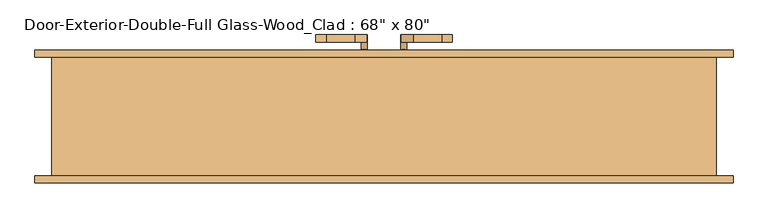
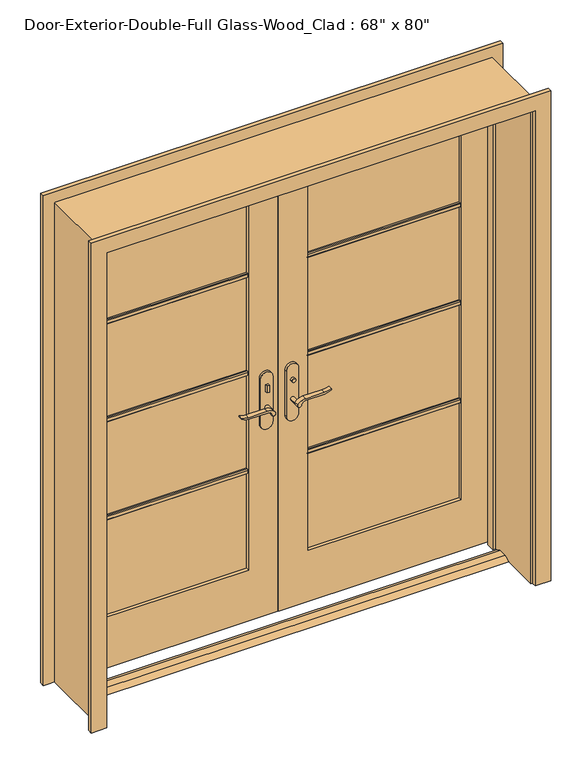
"""IFC4 building model written with IfcOpenShell, lengths in millimetres: door geometry."""

from ifc_helpers import new_model, si_unit, point, frame, frame_2d, origin, place, context, project, spatial, polyline, circle_curve, trimmed, segment, composite_curve, outline, extrude, faceted_brep, source, transform, mapped, element, save


def door_97aac55e(model_context):
    return source(origin(), model_context, "Body", "SolidModel", [
        extrude(outline(polyline([(19.05, 12.7), (53.975, 12.7), (79.375, 0.0), (-6.35, 0.0), (19.05, 12.7)])), frame((-863.6, 0.0, 0.0), z_axis=(1.0, 0.0, 0.0), x_axis=(0.0, 1.0, 0.0)), (0.0, 0.0, 1.0), 1727.2),
        extrude(outline(polyline([(-47.4019111, 100.65), (-57.4019111, 100.65), (-57.4019111, 110.65), (-47.4019111, 110.65), (-47.4019111, 100.65)])), frame((0.0, 0.0, 981.9), z_axis=(0.0, 0.0, 1.0), x_axis=(1.0, 0.0, 0.0)), (0.0, 0.0, 1.0), 30.0),
        extrude(outline(composite_curve([segment(trimmed(circle_curve(frame_2d((996.9, -52.4019111)), 8.0), [point((996.9, -60.4019111))], [point((996.9, -44.4019111))], False, "CARTESIAN"), True, "CONTINUOUS"), segment(trimmed(circle_curve(frame_2d((996.9, -52.4019111)), 8.0), [point((996.9, -44.4019111))], [point((996.9, -60.4019111))], False, "CARTESIAN"), True, "CONTINUOUS")], self_intersect=False)), frame((0.0, 165.575, 0.0), z_axis=(0.0, 1.0, 0.0), x_axis=(0.0, 0.0, 1.0)), (0.0, 0.0, 1.0), 10.0),
        extrude(outline(composite_curve([segment(trimmed(circle_curve(frame_2d((897.1555521, -76.0694241)), 37.2832219), [point((919.0523287, -45.8937749))], [point((934.4, -77.7693445))], False, "CARTESIAN"), True, "CONTINUOUS"), segment(polyline([(934.4, -77.7693445), (934.4, -154.045502)]), True, "CONTINUOUS"), segment(trimmed(circle_curve(frame_2d((1017.6850638, -153.9791202)), 83.2850902), [point((934.4, -154.045502))], [point((939.4, -182.4019111))], True, "CARTESIAN"), True, "CONTINUOUS"), segment(polyline([(939.4, -182.4019111), (936.6135558, -182.4019111)]), True, "CONTINUOUS"), segment(trimmed(circle_curve(frame_2d((986.6709207, -150.4622499)), 59.3791355), [point((936.6135558, -182.4019111))], [point((927.4, -154.045502))], False, "CARTESIAN"), True, "CONTINUOUS"), segment(polyline([(927.4, -154.045502), (927.4, -77.7881013)]), True, "CONTINUOUS"), segment(trimmed(circle_curve(frame_2d((909.2738613, -77.7881013)), 18.1261387), [point((927.4, -77.7881013))], [point((914.4, -60.4019111))], True, "CARTESIAN"), True, "CONTINUOUS"), segment(trimmed(circle_curve(frame_2d((914.4, -52.4019111)), 8.0), [point((914.4, -60.4019111))], [point((919.0523287, -45.8937749))], False, "CARTESIAN"), True, "CONTINUOUS")], self_intersect=False)), frame((0.0, 60.65, 0.0), z_axis=(0.0, 1.0, 0.0), x_axis=(0.0, 0.0, 1.0)), (0.0, 0.0, 1.0), 20.0),
        extrude(outline(composite_curve([segment(trimmed(circle_curve(frame_2d((914.4, -52.4019111)), 8.0), [point((914.3999903, -60.4019111))], [point((919.0523287, -45.8937749))], False, "CARTESIAN"), True, "CONTINUOUS"), segment(trimmed(circle_curve(frame_2d((897.1555521, -76.0694241)), 37.2832219), [point((919.0523287, -45.8937749))], [point((934.4, -77.7693445))], False, "CARTESIAN"), True, "CONTINUOUS"), segment(polyline([(934.4, -77.7693445), (934.4, -154.045502)]), True, "CONTINUOUS"), segment(trimmed(circle_curve(frame_2d((1017.6850638, -153.9791202)), 83.2850902), [point((934.4, -154.045502))], [point((939.4, -182.4019111))], True, "CARTESIAN"), True, "CONTINUOUS"), segment(polyline([(939.4, -182.4019111), (936.6135558, -182.4019111)]), True, "CONTINUOUS"), segment(trimmed(circle_curve(frame_2d((986.6709207, -150.4622499)), 59.3791355), [point((936.6135558, -182.4019111))], [point((927.4, -154.045502))], False, "CARTESIAN"), True, "CONTINUOUS"), segment(polyline([(927.4, -154.045502), (927.4, -77.788099)]), True, "CONTINUOUS"), segment(trimmed(circle_curve(frame_2d((909.2738682, -77.788099)), 18.1261318), [point((927.4, -77.788099))], [point((914.3999903, -60.4019111))], True, "CARTESIAN"), True, "CONTINUOUS")], self_intersect=False)), frame((0.0, 195.575, 0.0), z_axis=(0.0, 1.0, 0.0), x_axis=(0.0, 0.0, 1.0)), (0.0, 0.0, 1.0), 20.0),
        extrude(outline(composite_curve([segment(trimmed(circle_curve(frame_2d((914.4, -52.4019111)), 8.0), [point((914.4, -60.4019111))], [point((914.4, -44.4019111))], False, "CARTESIAN"), True, "CONTINUOUS"), segment(trimmed(circle_curve(frame_2d((914.4, -52.4019111)), 8.0), [point((914.4, -44.4019111))], [point((914.4, -60.4019111))], False, "CARTESIAN"), True, "CONTINUOUS")], self_intersect=False)), frame((0.0, 80.65, 0.0), z_axis=(0.0, 1.0, 0.0), x_axis=(0.0, 0.0, 1.0)), (0.0, 0.0, 1.0), 30.0),
        extrude(outline(composite_curve([segment(trimmed(circle_curve(frame_2d((914.4, -52.4019111)), 8.0), [point((914.4, -60.4019111))], [point((914.4, -44.4019111))], False, "CARTESIAN"), True, "CONTINUOUS"), segment(trimmed(circle_curve(frame_2d((914.4, -52.4019111)), 8.0), [point((914.4, -44.4019111))], [point((914.4, -60.4019111))], False, "CARTESIAN"), True, "CONTINUOUS")], self_intersect=False)), frame((0.0, 165.575, 0.0), z_axis=(0.0, 1.0, 0.0), x_axis=(0.0, 0.0, 1.0)), (0.0, 0.0, 1.0), 30.0),
        extrude(outline(composite_curve([segment(polyline([(844.4, -27.4019111), (1039.4, -27.4019111)]), True, "CONTINUOUS"), segment(trimmed(circle_curve(frame_2d((1039.4, -52.4019111)), 25.0), [point((1039.4, -27.4019111))], [point((1039.4, -77.4019111))], False, "CARTESIAN"), True, "CONTINUOUS"), segment(polyline([(1039.4, -77.4019111), (844.4, -77.4019111)]), True, "CONTINUOUS"), segment(trimmed(circle_curve(frame_2d((844.4, -52.4019111)), 25.0), [point((844.4, -77.4019111))], [point((844.4, -27.4019111))], False, "CARTESIAN"), True, "CONTINUOUS")], self_intersect=False)), frame((0.0, 110.65, 0.0), z_axis=(0.0, 1.0, 0.0), x_axis=(0.0, 0.0, 1.0)), (0.0, 0.0, 1.0), 10.0),
        extrude(outline(composite_curve([segment(polyline([(844.4, -27.4019111), (1039.4, -27.4019111)]), True, "CONTINUOUS"), segment(trimmed(circle_curve(frame_2d((1039.4, -52.4019111)), 25.0), [point((1039.4, -27.4019111))], [point((1039.4, -77.4019111))], False, "CARTESIAN"), True, "CONTINUOUS"), segment(polyline([(1039.4, -77.4019111), (844.4, -77.4019111)]), True, "CONTINUOUS"), segment(trimmed(circle_curve(frame_2d((844.4, -52.4019111)), 25.0), [point((844.4, -77.4019111))], [point((844.4, -27.4019111))], False, "CARTESIAN"), True, "CONTINUOUS")], self_intersect=False)), frame((0.0, 155.575, 0.0), z_axis=(0.0, 1.0, 0.0), x_axis=(0.0, 0.0, 1.0)), (0.0, 0.0, 1.0), 10.0),
        extrude(outline(polyline([(47.3875, 175.575), (57.3875, 175.575), (57.3875, 165.575), (47.3875, 165.575), (47.3875, 175.575)])), frame((0.0, 0.0, 981.9), z_axis=(0.0, 0.0, 1.0), x_axis=(1.0, 0.0, 0.0)), (0.0, 0.0, 1.0), 30.0),
        extrude(outline(composite_curve([segment(trimmed(circle_curve(frame_2d((996.9, 52.3875)), 8.0), [point((996.9, 60.3875))], [point((996.9, 44.3875))], False, "CARTESIAN"), True, "CONTINUOUS"), segment(trimmed(circle_curve(frame_2d((996.9, 52.3875)), 8.0), [point((996.9, 44.3875))], [point((996.9, 60.3875))], False, "CARTESIAN"), True, "CONTINUOUS")], self_intersect=False)), frame((0.0, 100.65, 0.0), z_axis=(0.0, 1.0, 0.0), x_axis=(0.0, 0.0, 1.0)), (0.0, 0.0, 1.0), 10.0),
        extrude(outline(composite_curve([segment(trimmed(circle_curve(frame_2d((914.4, 52.3875)), 8.0), [point((919.0523287, 45.8793637))], [point((914.4, 60.3875))], False, "CARTESIAN"), True, "CONTINUOUS"), segment(trimmed(circle_curve(frame_2d((909.2738613, 77.7736901)), 18.1261387), [point((914.4, 60.3875))], [point((927.4, 77.7736901))], True, "CARTESIAN"), True, "CONTINUOUS"), segment(polyline([(927.4, 77.7736901), (927.4, 154.0310909)]), True, "CONTINUOUS"), segment(trimmed(circle_curve(frame_2d((986.6709207, 150.4478388)), 59.3791355), [point((927.4, 154.0310909))], [point((936.6135558, 182.3875))], False, "CARTESIAN"), True, "CONTINUOUS"), segment(polyline([(936.6135558, 182.3875), (939.4, 182.3875)]), True, "CONTINUOUS"), segment(trimmed(circle_curve(frame_2d((1017.6850638, 153.9647091)), 83.2850902), [point((939.4, 182.3875))], [point((934.4, 154.0310909))], True, "CARTESIAN"), True, "CONTINUOUS"), segment(polyline([(934.4, 154.0310909), (934.4, 77.7549333)]), True, "CONTINUOUS"), segment(trimmed(circle_curve(frame_2d((897.1555521, 76.0550129)), 37.2832219), [point((934.4, 77.7549333))], [point((919.0523287, 45.8793637))], False, "CARTESIAN"), True, "CONTINUOUS")], self_intersect=False)), frame((0.0, 195.575, 0.0), z_axis=(0.0, 1.0, 0.0), x_axis=(0.0, 0.0, 1.0)), (0.0, 0.0, 1.0), 20.0),
        extrude(outline(composite_curve([segment(trimmed(circle_curve(frame_2d((909.2738682, 77.7736878)), 18.1261318), [point((914.3999903, 60.3875))], [point((927.4, 77.7736878))], True, "CARTESIAN"), True, "CONTINUOUS"), segment(polyline([(927.4, 77.7736878), (927.4, 154.0310909)]), True, "CONTINUOUS"), segment(trimmed(circle_curve(frame_2d((986.6709207, 150.4478388)), 59.3791355), [point((927.4, 154.0310909))], [point((936.6135558, 182.3875))], False, "CARTESIAN"), True, "CONTINUOUS"), segment(polyline([(936.6135558, 182.3875), (939.4, 182.3875)]), True, "CONTINUOUS"), segment(trimmed(circle_curve(frame_2d((1017.6850638, 153.9647091)), 83.2850902), [point((939.4, 182.3875))], [point((934.4, 154.0310909))], True, "CARTESIAN"), True, "CONTINUOUS"), segment(polyline([(934.4, 154.0310909), (934.4, 77.7549333)]), True, "CONTINUOUS"), segment(trimmed(circle_curve(frame_2d((897.1555521, 76.0550129)), 37.2832219), [point((934.4, 77.7549333))], [point((919.0523287, 45.8793637))], False, "CARTESIAN"), True, "CONTINUOUS"), segment(trimmed(circle_curve(frame_2d((914.4, 52.3875)), 8.0), [point((919.0523287, 45.8793637))], [point((914.3999903, 60.3875))], False, "CARTESIAN"), True, "CONTINUOUS")], self_intersect=False)), frame((0.0, 60.65, 0.0), z_axis=(0.0, 1.0, 0.0), x_axis=(0.0, 0.0, 1.0)), (0.0, 0.0, 1.0), 20.0),
        extrude(outline(composite_curve([segment(trimmed(circle_curve(frame_2d((914.4, 52.3875)), 8.0), [point((914.4, 60.3875))], [point((914.4, 44.3875))], False, "CARTESIAN"), True, "CONTINUOUS"), segment(trimmed(circle_curve(frame_2d((914.4, 52.3875)), 8.0), [point((914.4, 44.3875))], [point((914.4, 60.3875))], False, "CARTESIAN"), True, "CONTINUOUS")], self_intersect=False)), frame((0.0, 165.575, 0.0), z_axis=(0.0, 1.0, 0.0), x_axis=(0.0, 0.0, 1.0)), (0.0, 0.0, 1.0), 30.0),
        extrude(outline(composite_curve([segment(trimmed(circle_curve(frame_2d((914.4, 52.3875)), 8.0), [point((914.4, 60.3875))], [point((914.4, 44.3875))], False, "CARTESIAN"), True, "CONTINUOUS"), segment(trimmed(circle_curve(frame_2d((914.4, 52.3875)), 8.0), [point((914.4, 44.3875))], [point((914.4, 60.3875))], False, "CARTESIAN"), True, "CONTINUOUS")], self_intersect=False)), frame((0.0, 80.65, 0.0), z_axis=(0.0, 1.0, 0.0), x_axis=(0.0, 0.0, 1.0)), (0.0, 0.0, 1.0), 30.0),
        extrude(outline(composite_curve([segment(trimmed(circle_curve(frame_2d((844.4, 52.3875)), 25.0), [point((844.4, 27.3875))], [point((844.4, 77.3875))], False, "CARTESIAN"), True, "CONTINUOUS"), segment(polyline([(844.4, 77.3875), (1039.4, 77.3875)]), True, "CONTINUOUS"), segment(trimmed(circle_curve(frame_2d((1039.4, 52.3875)), 25.0), [point((1039.4, 77.3875))], [point((1039.4, 27.3875))], False, "CARTESIAN"), True, "CONTINUOUS"), segment(polyline([(1039.4, 27.3875), (844.4, 27.3875)]), True, "CONTINUOUS")], self_intersect=False)), frame((0.0, 155.575, 0.0), z_axis=(0.0, 1.0, 0.0), x_axis=(0.0, 0.0, 1.0)), (0.0, 0.0, 1.0), 10.0),
        extrude(outline(composite_curve([segment(trimmed(circle_curve(frame_2d((844.4, 52.3875)), 25.0), [point((844.4, 27.3875))], [point((844.4, 77.3875))], False, "CARTESIAN"), True, "CONTINUOUS"), segment(polyline([(844.4, 77.3875), (1039.4, 77.3875)]), True, "CONTINUOUS"), segment(trimmed(circle_curve(frame_2d((1039.4, 52.3875)), 25.0), [point((1039.4, 77.3875))], [point((1039.4, 27.3875))], False, "CARTESIAN"), True, "CONTINUOUS"), segment(polyline([(1039.4, 27.3875), (844.4, 27.3875)]), True, "CONTINUOUS")], self_intersect=False)), frame((0.0, 110.65, 0.0), z_axis=(0.0, 1.0, 0.0), x_axis=(0.0, 0.0, 1.0)), (0.0, 0.0, 1.0), 10.0),
        extrude(outline(polyline([(134.62, 1502.171875), (134.62, 1483.121875), (128.27, 1483.121875), (125.095, 1486.296875), (125.095, 1498.996875), (128.27, 1502.171875), (134.62, 1502.171875)])), frame((120.65, 0.0, 0.0), z_axis=(1.0, 0.0, 0.0), x_axis=(0.0, 1.0, 0.0)), (0.0, 0.0, 1.0), 622.3),
        extrude(outline(polyline([(134.62, 1081.88125), (134.62, 1062.83125), (128.27, 1062.83125), (125.095, 1066.00625), (125.095, 1078.70625), (128.27, 1081.88125), (134.62, 1081.88125)])), frame((120.65, 0.0, 0.0), z_axis=(1.0, 0.0, 0.0), x_axis=(0.0, 1.0, 0.0)), (0.0, 0.0, 1.0), 622.3),
        extrude(outline(polyline([(134.62, 661.590625), (134.62, 642.540625), (128.27, 642.540625), (125.095, 645.715625), (125.095, 658.415625), (128.27, 661.590625), (134.62, 661.590625)])), frame((120.65, 0.0, 0.0), z_axis=(1.0, 0.0, 0.0), x_axis=(0.0, 1.0, 0.0)), (0.0, 0.0, 1.0), 622.3),
        extrude(outline(polyline([(141.605, 1502.171875), (147.955, 1502.171875), (151.13, 1498.996875), (151.13, 1486.296875), (147.955, 1483.121875), (141.605, 1483.121875), (141.605, 1502.171875)])), frame((-742.95, 0.0, 0.0), z_axis=(1.0, 0.0, 0.0), x_axis=(0.0, 1.0, 0.0)), (0.0, 0.0, 1.0), 622.3),
        extrude(outline(polyline([(141.605, 1081.88125), (147.955, 1081.88125), (151.13, 1078.70625), (151.13, 1066.00625), (147.955, 1062.83125), (141.605, 1062.83125), (141.605, 1081.88125)])), frame((-742.95, 0.0, 0.0), z_axis=(1.0, 0.0, 0.0), x_axis=(0.0, 1.0, 0.0)), (0.0, 0.0, 1.0), 622.3),
        extrude(outline(polyline([(141.605, 661.590625), (147.955, 661.590625), (151.13, 658.415625), (151.13, 645.715625), (147.955, 642.540625), (141.605, 642.540625), (141.605, 661.590625)])), frame((-742.95, 0.0, 0.0), z_axis=(1.0, 0.0, 0.0), x_axis=(0.0, 1.0, 0.0)), (0.0, 0.0, 1.0), 622.3),
        extrude(outline(polyline([(141.605, 1502.171875), (147.955, 1502.171875), (151.13, 1498.996875), (151.13, 1486.296875), (147.955, 1483.121875), (141.605, 1483.121875), (141.605, 1502.171875)])), frame((120.65, 0.0, 0.0), z_axis=(1.0, 0.0, 0.0), x_axis=(0.0, 1.0, 0.0)), (0.0, 0.0, 1.0), 622.3),
        extrude(outline(polyline([(141.605, 1081.88125), (147.955, 1081.88125), (151.13, 1078.70625), (151.13, 1066.00625), (147.955, 1062.83125), (141.605, 1062.83125), (141.605, 1081.88125)])), frame((120.65, 0.0, 0.0), z_axis=(1.0, 0.0, 0.0), x_axis=(0.0, 1.0, 0.0)), (0.0, 0.0, 1.0), 622.3),
        extrude(outline(polyline([(141.605, 661.590625), (147.955, 661.590625), (151.13, 658.415625), (151.13, 645.715625), (147.955, 642.540625), (141.605, 642.540625), (141.605, 661.590625)])), frame((120.65, 0.0, 0.0), z_axis=(1.0, 0.0, 0.0), x_axis=(0.0, 1.0, 0.0)), (0.0, 0.0, 1.0), 622.3),
        extrude(outline(polyline([(134.62, 1502.171875), (134.62, 1483.121875), (128.27, 1483.121875), (125.095, 1486.296875), (125.095, 1498.996875), (128.27, 1502.171875), (134.62, 1502.171875)])), frame((-742.95, 0.0, 0.0), z_axis=(1.0, 0.0, 0.0), x_axis=(0.0, 1.0, 0.0)), (0.0, 0.0, 1.0), 622.3),
        extrude(outline(polyline([(134.62, 1081.88125), (134.62, 1062.83125), (128.27, 1062.83125), (125.095, 1066.00625), (125.095, 1078.70625), (128.27, 1081.88125), (134.62, 1081.88125)])), frame((-742.95, 0.0, 0.0), z_axis=(1.0, 0.0, 0.0), x_axis=(0.0, 1.0, 0.0)), (0.0, 0.0, 1.0), 622.3),
        extrude(outline(polyline([(134.62, 661.590625), (134.62, 642.540625), (128.27, 642.540625), (125.095, 645.715625), (125.095, 658.415625), (128.27, 661.590625), (134.62, 661.590625)])), frame((-742.95, 0.0, 0.0), z_axis=(1.0, 0.0, 0.0), x_axis=(0.0, 1.0, 0.0)), (0.0, 0.0, 1.0), 622.3),
        extrude(outline(polyline([(0.0, 869.95), (0.0, 933.45), (2101.85, 933.45), (2101.85, -933.45), (0.0, -933.45), (0.0, -869.95), (2038.35, -869.95), (2038.35, 869.95), (0.0, 869.95)])), frame((0.0, 155.575, 0.0), z_axis=(0.0, 1.0, 0.0), x_axis=(0.0, 0.0, 1.0)), (0.0, 0.0, 1.0), 19.05),
        extrude(outline(polyline([(0.0, 869.95), (0.0, 933.45), (2101.85, 933.45), (2101.85, -933.45), (0.0, -933.45), (0.0, -869.95), (2038.35, -869.95), (2038.35, 869.95), (0.0, 869.95)])), frame((0.0, -180.975, 0.0), z_axis=(0.0, 1.0, 0.0), x_axis=(0.0, 0.0, 1.0)), (0.0, 0.0, 1.0), 19.05),
        extrude(outline(polyline([(12.7, 863.6), (2032.0, 863.6), (2032.0, 1.5875), (12.7, 1.5875), (12.7, 863.6)]), holes=[polyline([(1912.9375, 120.65), (1912.9375, 742.95), (231.775, 742.95), (231.775, 120.65), (1912.9375, 120.65)])]), frame((0.0, 120.65, 0.0), z_axis=(0.0, 1.0, 0.0), x_axis=(0.0, 0.0, 1.0)), (0.0, 0.0, 1.0), 34.925),
        extrude(outline(polyline([(2032.0, -863.6), (12.7, -863.6), (12.7, -1.6019111), (2032.0, -1.6019111), (2032.0, -863.6)]), holes=[polyline([(231.775, -742.95), (1912.9375, -742.95), (1912.9375, -120.65), (231.775, -120.65), (231.775, -742.95)])]), frame((0.0, 120.65, 0.0), z_axis=(0.0, 1.0, 0.0), x_axis=(0.0, 0.0, 1.0)), (0.0, 0.0, 1.0), 34.925),
        faceted_brep([(889.0, 155.575, 0.0), (889.0, -161.925, 0.0), (863.6, -161.925, 0.0), (863.6, 85.725, 0.0), (850.9, 85.725, 0.0), (850.9, 120.65, 0.0), (863.6, 120.65, 0.0), (863.6, 155.575, 0.0), (889.0, 155.575, 2057.4), (889.0, -161.925, 2057.4), (-889.0, -161.925, 2057.4), (-889.0, -161.925, 0.0), (-863.6, -161.925, 0.0), (-863.6, -161.925, 2032.0), (863.6, -161.925, 2032.0), (863.6, 85.725, 2032.0), (-863.6, 85.725, 2032.0), (-863.6, 85.725, 0.0), (-850.9, 85.725, 0.0), (-850.9, 85.725, 2019.3), (850.9, 85.725, 2019.3), (850.9, 120.65, 2019.3), (1.5875, 120.65, 2019.3), (-1.6019111, 120.65, 2019.3), (-850.9, 120.65, 2019.3), (-850.9, 120.65, 0.0), (-863.6, 120.65, 0.0), (-863.6, 120.65, 2032.0), (-1.6019111, 120.65, 2032.0), (1.5875, 120.65, 2032.0), (863.6, 120.65, 2032.0), (863.6, 155.575, 2032.0), (1.5875, 155.575, 2032.0), (-1.6019111, 155.575, 2032.0), (-863.6, 155.575, 2032.0), (-863.6, 155.575, 0.0), (-889.0, 155.575, 0.0), (-889.0, 155.575, 2057.4)], [[[0, 1, 2, 3, 4, 5, 6, 7]], [[1, 0, 8, 9]], [[2, 1, 9, 10, 11, 12, 13, 14]], [[3, 2, 14, 15]], [[4, 3, 15, 16, 17, 18, 19, 20]], [[5, 4, 20, 21]], [[6, 5, 21, 22, 23, 24, 25, 26, 27, 28, 29, 30]], [[7, 6, 30, 31]], [[0, 7, 31, 32, 33, 34, 35, 36, 37, 8]], [[9, 8, 37, 10]], [[14, 13, 16, 15]], [[20, 19, 24, 23, 22, 21]], [[31, 30, 29, 28, 27, 34, 33, 32]], [[12, 11, 36, 35, 26, 25, 18, 17]], [[11, 10, 37, 36]], [[13, 12, 17, 16]], [[19, 18, 25, 24]], [[27, 26, 35, 34]]]),
        extrude(outline(polyline([(742.95, 134.62), (120.65, 134.62), (120.65, 141.605), (742.95, 141.605), (742.95, 134.62)])), frame((0.0, 0.0, 231.775), z_axis=(0.0, 0.0, 1.0), x_axis=(1.0, 0.0, 0.0)), (0.0, 0.0, 1.0), 1681.1625),
        extrude(outline(polyline([(-120.65, 134.62), (-742.95, 134.62), (-742.95, 141.605), (-120.65, 141.605), (-120.65, 134.62)])), frame((0.0, 0.0, 231.775), z_axis=(0.0, 0.0, 1.0), x_axis=(1.0, 0.0, 0.0)), (0.0, 0.0, 1.0), 1681.1625),
    ])


if __name__ == "__main__":
    model = new_model("IFC4")
    model_context = context("Model", 3, world=origin())
    ifc_project = project(units=[si_unit("LENGTHUNIT", "METRE", prefix="MILLI")], contexts=[model_context])
    site = spatial("IfcSite", under=ifc_project)
    building = spatial("IfcBuilding", under=site)
    placement = place(None, origin())
    door_shape = door_97aac55e(model_context)
    element("IfcDoor", 1, ObjectType="Door-Exterior-Double-Full Glass-Wood_Clad : 68\" x 80\"", at=placement, inside=building, context=model_context, shape_type="MappedRepresentation", body=[
        mapped(door_shape, transform((0.0, 0.0, 0.0), x_axis=(1.0, 0.0, 0.0), y_axis=(0.0, 1.0, 0.0), z_axis=(0.0, 0.0, 1.0))),
    ])
    save(model, "model.ifc")

# Revit data of these elements
# Type "Door-Exterior-Double-Full Glass-Wood_Clad : 68\" x 80\""
#   Type Mark = "21"
#   Assembly Code = "B2030100"
#   Analytic Construction = "French door, wood frame with double glass"
#   Top Rail = 0' - 4 11/16"
#   Threshold Offset [instance default] = 0' - 0 1/2"
#   Thickness = 0' - 1 3/8"
#   Thermal Resistance (R) = 1.9158 (h·ft²·°F)/BTU
#   Swing Angle [instance default] = 90.0000°
#   Stiles = 0' - 4 3/4"
#   Rough Width = 5' - 10"
#   Rough Height = 6' - 9"
#   Panel Width = 2' - 10"
#   Door Offset [instance default] = 0' - 0"
#   Height = 6' - 8"
#   Width = 5' - 8"
#   Heat Transfer Coefficient (U) = 0.5220 BTU/(h·ft²·°F)
#   Bottom Rail = 0' - 9 1/8"
#   Exterior Trim [instance default] = yes
#   Threshold [instance default] = yes
#   Show Grill [instance default] = yes
#   Function = 1
#   Trim Material = Clad - White
#   Threshold Material = Maple - Semigloss(Rotated)
#   Panel Material = Clad - White
#   Glazing = Glass, Clear Glazing
#   Frame Material = Clad - White
#   Door Handle Material = Aluminum
#   Visual Light Transmittance = 0
#   Solar Heat Gain Coefficient = 0
#   Wall Closure = (empty or 0)
#   Construction Type = (empty or 0)
# Element 1 (IfcDoor, "Door-Exterior-Double-Full Glass-Wood_Clad : 68\" x 80\"")
#   Materials on its faces: "Clad - White", "Aluminum", "Glass, Clear Glazing", "Maple - Semigloss(Rotated)"
# Materials
#   "Clad - White": class "Wood", colour RGB 245 245 243, transparency 0, Cost = 0
#   "Maple - Semigloss(Rotated)": class "Wood", colour RGB 196 161 118, transparency 0, Description = "Acer Saccharum", Cost = 0
#   "Glass, Clear Glazing": class "Glass", colour RGB 245 245 243, transparency 1, Description = "Clear glazing", Cost = 0
#   "Aluminum": class "Metal", colour RGB 244 245 246, transparency 0, Description = "Aluminum 6061", Cost = 0
